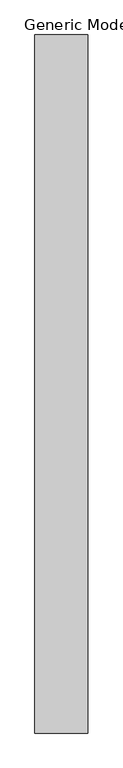
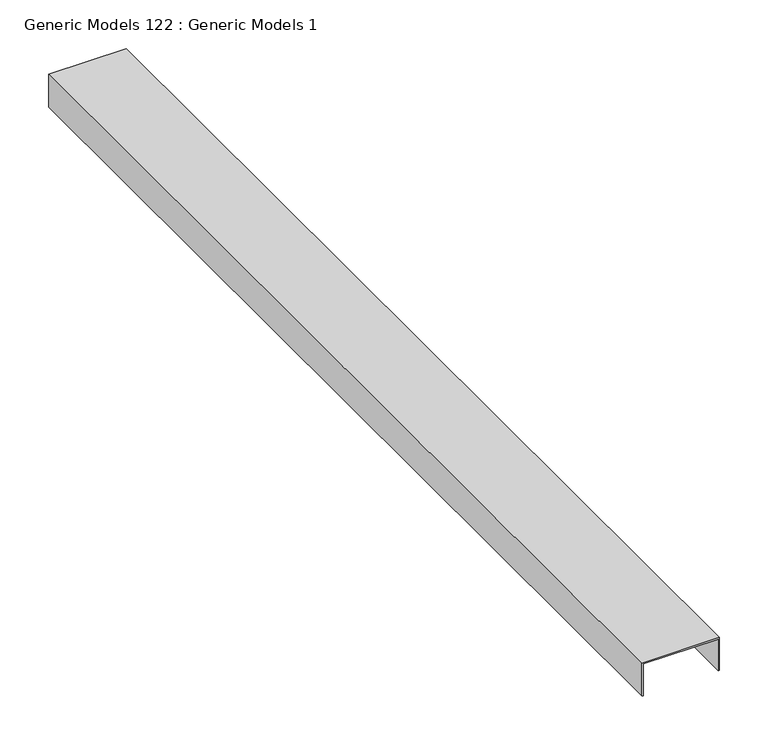
"""IFC4 building model written with IfcOpenShell, lengths in millimetres: proxy geometry, Generic Models 122 : Generic Models 1."""

import ifcopenshell
import ifcopenshell.guid

model = None  # the IFC model being written
_history = None  # IfcOwnerHistory: only IFC2X3 demands one
_inside = {}  # id of a spatial element -> (the spatial element, [elements in it])
_under = {}  # id of a project, library or spatial element -> (it, [spatial elements below it])
_declared = {}  # id of a project -> (the project, [libraries it declares])
_typed = {}  # id of a type object -> (the type object, [elements of that type])
_made_of = {}  # id of a material, layer set ... -> (it, [elements and type objects made of it])


def new_model(schema):
    """Start an empty IFC model of exactly this schema.

    Asked for "IFC4X3", IfcOpenShell would pick the latest addendum, in which some entities
    have other attributes; the version numbers below select the first issue.
    IFC2X3 requires an IfcOwnerHistory on every rooted entity: one is made here for all.
    """
    global model, _history
    if schema == "IFC4X3":
        model = ifcopenshell.file(schema_version=(4, 3, 0, 0))
    else:
        model = ifcopenshell.file(schema=schema)
    _inside.clear()
    _under.clear()
    _declared.clear()
    _typed.clear()
    _made_of.clear()
    _history = None
    if model.schema == "IFC2X3":
        org = make("IfcOrganization", Name="unknown")
        user = make(
            "IfcPersonAndOrganization",
            ThePerson=make("IfcPerson", FamilyName="unknown"),
            TheOrganization=org,
        )
        app = make(
            "IfcApplication",
            ApplicationDeveloper=org,
            Version="unknown",
            ApplicationFullName="unknown",
            ApplicationIdentifier="unknown",
        )
        _history = make(
            "IfcOwnerHistory",
            OwningUser=user,
            OwningApplication=app,
            ChangeAction="ADDED",
            CreationDate=0,
        )
    return model


def make(cls, **values):
    """One entity of the class cls with the attributes given. An attribute that is None is left unset."""
    return model.create_entity(
        cls, **{name: value for name, value in values.items() if value is not None}
    )


def rooted(cls, **values):
    """An entity with a GlobalId (a new one), such as an element, a storey or a relation."""
    return make(cls, GlobalId=ifcopenshell.guid.new(), OwnerHistory=_history, **values)


def si_unit(unit_type, name, prefix=None):
    """IfcSIUnit, for example si_unit("LENGTHUNIT", "METRE", prefix="MILLI")."""
    return make("IfcSIUnit", UnitType=unit_type, Prefix=prefix, Name=name)


def assignment(units):
    """IfcUnitAssignment: the units of a project."""
    return None if units is None else make("IfcUnitAssignment", Units=units)


def point(xyz):
    """IfcCartesianPoint."""
    return None if xyz is None else make("IfcCartesianPoint", Coordinates=xyz)


def direction(xyz):
    """IfcDirection."""
    return None if xyz is None else make("IfcDirection", DirectionRatios=xyz)


def frame(location, z_axis=None, x_axis=None):
    """IfcAxis2Placement3D, a coordinate frame: its origin and axes. An axis left out is left unset."""
    return make(
        "IfcAxis2Placement3D",
        Location=point(location),
        Axis=direction(z_axis),
        RefDirection=direction(x_axis),
    )


def origin():
    """The frame at (0, 0, 0) with its axes left unset."""
    return frame((0.0, 0.0, 0.0))


def place(relative_to, where):
    """IfcLocalPlacement: puts the frame where relative to a parent placement (None: the world)."""
    return make(
        "IfcLocalPlacement", PlacementRelTo=relative_to, RelativePlacement=where
    )


def context(
    kind, dimensions, precision=None, world=None, true_north=None, identifier=None
):
    """IfcGeometricRepresentationContext, for example the 3D "Model" context."""
    return make(
        "IfcGeometricRepresentationContext",
        ContextIdentifier=identifier,
        ContextType=kind,
        CoordinateSpaceDimension=dimensions,
        Precision=precision,
        WorldCoordinateSystem=world,
        TrueNorth=true_north,
    )


def project(units=None, contexts=None):
    """IfcProject with its units and contexts."""
    return rooted(
        "IfcProject",
        Name="project",
        RepresentationContexts=contexts,
        UnitsInContext=assignment(units),
    )


def spatial(cls, under=None, at=None, **own):
    """A site, building, storey or space (cls), placed at a placement, below another one or the project."""
    s = rooted(cls, ObjectPlacement=at, **own)
    if under is not None:
        _under.setdefault(under.id(), (under, []))[1].append(s)
    return s


def polyline(points):
    """IfcPolyline through the points."""
    return make("IfcPolyline", Points=[point(p) for p in points])


def outline(outer, holes=None, kind="AREA"):
    """IfcArbitraryClosedProfileDef: a profile drawn as a closed curve; with holes, ...WithVoids."""
    if holes is None:
        return make("IfcArbitraryClosedProfileDef", ProfileType=kind, OuterCurve=outer)
    return make(
        "IfcArbitraryProfileDefWithVoids",
        ProfileType=kind,
        OuterCurve=outer,
        InnerCurves=holes,
    )


def extrude(swept, where, along, depth):
    """IfcExtrudedAreaSolid: the profile swept, set in the frame where, extruded along a direction by depth."""
    return make(
        "IfcExtrudedAreaSolid",
        SweptArea=swept,
        Position=where,
        ExtrudedDirection=direction(along),
        Depth=depth,
    )


def shape(context_of_items, identifier, shape_type, items):
    """IfcShapeRepresentation: the items that make up one representation, for example the "Body"."""
    return make(
        "IfcShapeRepresentation",
        ContextOfItems=context_of_items,
        RepresentationIdentifier=identifier,
        RepresentationType=shape_type,
        Items=items,
    )


def source(mapping_origin, context_of_items, identifier, shape_type, items):
    """IfcRepresentationMap: a shape defined once, which mapped items show again and again."""
    return make(
        "IfcRepresentationMap",
        MappingOrigin=mapping_origin,
        MappedRepresentation=shape(context_of_items, identifier, shape_type, items),
    )


def transform(
    local_origin,
    x_axis=None,
    y_axis=None,
    z_axis=None,
    scale=None,
    scale2=None,
    scale3=None,
    uniform=True,
):
    """IfcCartesianTransformationOperator3D, or its non-uniform kind. x_axis, y_axis, z_axis: its Axis1, 2, 3."""
    if uniform:
        return make(
            "IfcCartesianTransformationOperator3D",
            Axis1=direction(x_axis),
            Axis2=direction(y_axis),
            LocalOrigin=point(local_origin),
            Scale=scale,
            Axis3=direction(z_axis),
        )
    return make(
        "IfcCartesianTransformationOperator3DnonUniform",
        Axis1=direction(x_axis),
        Axis2=direction(y_axis),
        LocalOrigin=point(local_origin),
        Scale=scale,
        Axis3=direction(z_axis),
        Scale2=scale2,
        Scale3=scale3,
    )


def mapped(mapping_source, mapping_target):
    """IfcMappedItem: shows the shape of a source again, moved by a transform."""
    return make(
        "IfcMappedItem", MappingSource=mapping_source, MappingTarget=mapping_target
    )


def made_of(thing, what):
    """Note that an element or type object is made of a material, layer set ...; save() writes the relation."""
    if what is not None:
        _made_of.setdefault(what.id(), (what, []))[1].append(thing)
    return thing


def element(
    cls,
    number,
    at=None,
    inside=None,
    cuts=None,
    type_object=None,
    material=None,
    context=None,
    identifier="Body",
    shape_type=None,
    held_by="IfcProductDefinitionShape",
    body=None,
    shapes=None,
    **own,
):
    """One element of the class cls, such as IfcWall. Its Tag is "e" and its number.

    at: its placement. inside: the storey or other place that contains it. cuts: it is an
    opening in that element (IfcRelVoidsElement). A single representation is given by context,
    identifier, shape_type and body (its items); several are given by shapes. held_by: the class
    of the entity that holds the representations. save() writes the other relations.
    """
    e = rooted(cls, Tag="e%d" % number, ObjectPlacement=at, **own)
    if body is not None:
        shapes = [shape(context, identifier, shape_type, body)]
    if shapes is not None:
        e.Representation = make(held_by, Representations=shapes)
    if inside is not None:
        _inside.setdefault(inside.id(), (inside, []))[1].append(e)
    if cuts is not None:
        rooted(
            "IfcRelVoidsElement", RelatingBuildingElement=cuts, RelatedOpeningElement=e
        )
    if type_object is not None:
        _typed.setdefault(type_object.id(), (type_object, []))[1].append(e)
    return made_of(e, material)


def aggregate(whole, parts):
    """IfcRelAggregates: a whole, such as a stair, and the parts it consists of."""
    return rooted("IfcRelAggregates", RelatingObject=whole, RelatedObjects=parts)


def save(model, path):
    """Write the relations noted so far, then the file.

    IfcRelAggregates (storeys below a building ...), IfcRelContainedInSpatialStructure (elements
    in a storey), IfcRelDefinesByType, IfcRelAssociatesMaterial and IfcRelDeclares: one each for
    every whole, place, type object, material and project.
    """
    for whole, parts in _under.values():
        aggregate(whole, parts)
    for where, things in _inside.values():
        rooted(
            "IfcRelContainedInSpatialStructure",
            RelatedElements=things,
            RelatingStructure=where,
        )
    for kind, things in _typed.values():
        rooted("IfcRelDefinesByType", RelatedObjects=things, RelatingType=kind)
    for what, things in _made_of.values():
        rooted("IfcRelAssociatesMaterial", RelatedObjects=things, RelatingMaterial=what)
    for by, libraries in _declared.values():
        rooted("IfcRelDeclares", RelatingContext=by, RelatedDefinitions=libraries)
    model.write(path)


def generic_models_122_generic_models_1_7f98dd7d(model_context):
    return source(origin(), model_context, "Body", "SweptSolid", [
        extrude(outline(polyline([(2231.473933, 46935.8735531), (2231.473933, 46843.7985531), (2190.198933, 46843.7985531), (2190.198933, 46845.3860531), (2229.886433, 46845.3860531), (2229.886433, 46934.2860531), (2190.198933, 46934.2860531), (2190.198933, 46935.8735531), (2231.473933, 46935.8735531)])), frame((0.0, 0.0, 0.0), z_axis=(0.0, 1.0, 0.0), x_axis=(0.0, 0.0, 1.0)), (0.0, 0.0, 1.0), 1219.2),
    ])


if __name__ == "__main__":
    model = new_model("IFC4")
    model_context = context("Model", 3, world=origin())
    ifc_project = project(units=[si_unit("LENGTHUNIT", "METRE", prefix="MILLI")], contexts=[model_context])
    site = spatial("IfcSite", under=ifc_project)
    building = spatial("IfcBuilding", under=site)
    placement = place(None, origin())
    generic_models_122_generic_models_1_shape = generic_models_122_generic_models_1_7f98dd7d(model_context)
    element("IfcBuildingElementProxy", 1, Name="Generic Models 122 : Generic Models 1", ObjectType="Generic Models 122 : Generic Models 1", at=placement, inside=building, context=model_context, shape_type="MappedRepresentation", body=[
        mapped(generic_models_122_generic_models_1_shape, transform((0.0, 0.0, 0.0), x_axis=(1.0, 0.0, 0.0), y_axis=(0.0, 1.0, 0.0), z_axis=(0.0, 0.0, 1.0))),
    ])
    save(model, "model.ifc")

# Revit data of these elements
# Element 1 (IfcBuildingElementProxy, "Generic Models 122 : Generic Models 1")
#   Materials on its faces: "DEEP LEG OF DEFLECTION TRACK (2\" MIN. DEFLECTION)"
# Materials
#   "DEEP LEG OF DEFLECTION TRACK (2\" MIN. DEFLECTION)": class "Unassigned", colour RGB 210 209 208, transparency 0, Keynote = "M05121300.02", Cost = 0
